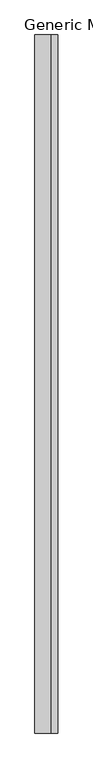
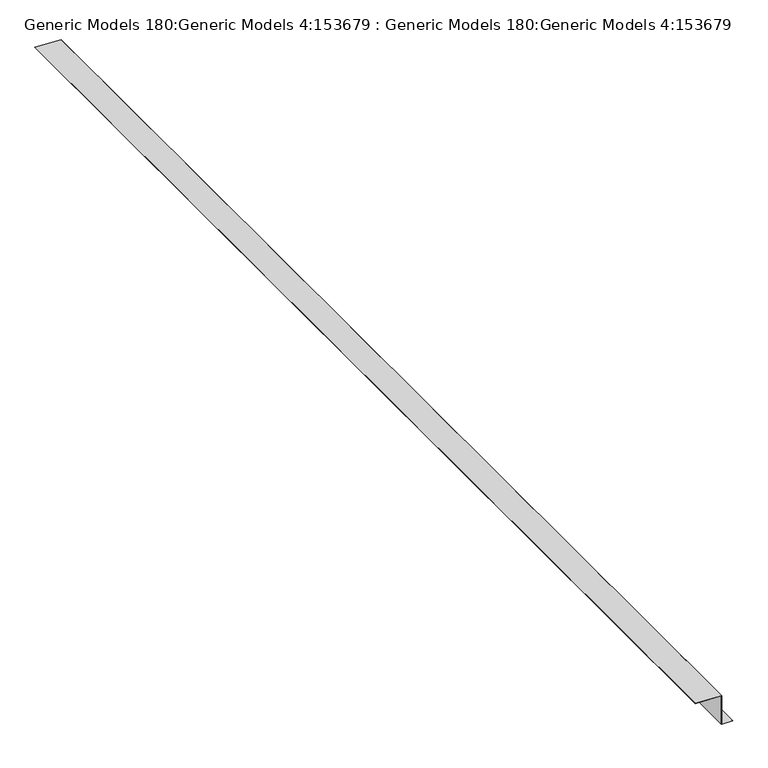
"""IFC4 building model written with IfcOpenShell, lengths in millimetres: proxy geometry, Generic Models 180:Generic Models 4:153679 : Generic Models 180:Generic Models 4:153679."""

from ifc_helpers import new_model, si_unit, frame, origin, place, context, project, spatial, polyline, outline, extrude, source, transform, mapped, element, save


def generic_models_180_generic_models_4_153679_generic_models_0acd0943(model_context):
    return source(origin(), model_context, "Body", "SweptSolid", [
        extrude(outline(polyline([(3632.2816052, -8378.8756261), (3625.128051, -8206.7030369), (3428.0607838, -8206.7030369), (3426.7471943, -8131.4475458), (3427.5408234, -8131.4336929), (3428.8407998, -8205.9092869), (3625.8895065, -8205.9092869), (3633.0746709, -8378.8426752), (3632.2816052, -8378.8756261)])), frame((0.0, -273.9974793, 0.0), z_axis=(0.0, 1.0, 0.0), x_axis=(0.0, 0.0, 1.0)), (0.0, 0.0, 1.0), 7518.4),
    ])


if __name__ == "__main__":
    model = new_model("IFC4")
    model_context = context("Model", 3, world=origin())
    ifc_project = project(units=[si_unit("LENGTHUNIT", "METRE", prefix="MILLI")], contexts=[model_context])
    site = spatial("IfcSite", under=ifc_project)
    building = spatial("IfcBuilding", under=site)
    placement = place(None, origin())
    generic_models_180_generic_models_4_153679_generic_models_shape = generic_models_180_generic_models_4_153679_generic_models_0acd0943(model_context)
    element("IfcBuildingElementProxy", 1, Name="Generic Models 180:Generic Models 4:153679 : Generic Models 180:Generic Models 4:153679", ObjectType="Generic Models 180:Generic Models 4:153679 : Generic Models 180:Generic Models 4:153679", at=placement, inside=building, context=model_context, shape_type="MappedRepresentation", body=[
        mapped(generic_models_180_generic_models_4_153679_generic_models_shape, transform((0.0, 0.0, 0.0), x_axis=(1.0, 0.0, 0.0), y_axis=(0.0, 1.0, 0.0), z_axis=(0.0, 0.0, 1.0))),
    ])
    save(model, "model.ifc")

# Revit data of these elements
# Type "Generic Models 180:Generic Models 4:153679 : Generic Models 180:Generic Models 4:153679"
#   NameOverride = "Generic Models 180:Generic Models 4:153679"
#   ObjectTypeOverride = "Generic Models 180:Generic Models 4"
#   Reference = "Generic Models 4"
#   Category = "Generic Models"
#   Tag = "153679"
# Element 1 (IfcBuildingElementProxy, "Generic Models 180:Generic Models 4:153679 : Generic Models 180:Generic Models 4:153679")
#   Materials on its faces: "_HYDROSTOP LIQUID MEMBRANE -FOLLOW MANU. RECOMMENDED INSTALLATION DETAILS 15173"
# Materials
#   "_HYDROSTOP LIQUID MEMBRANE -FOLLOW MANU. RECOMMENDED INSTALLATION DETAILS 15173": class "Unassigned", colour RGB 100 140 119, transparency 0
